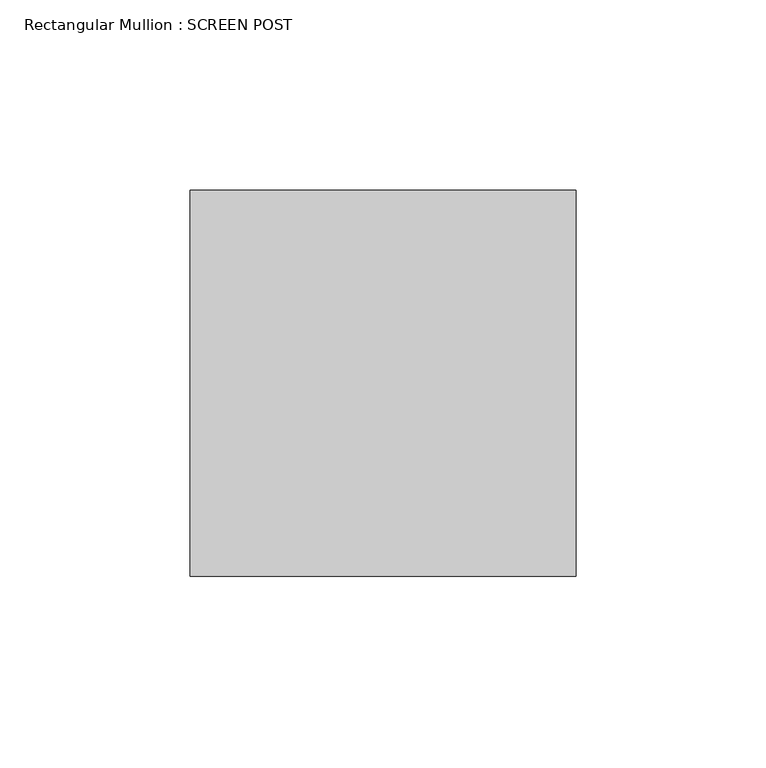
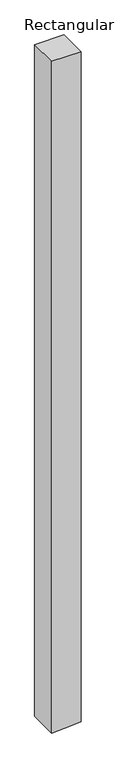
"""IFC4 building model written with IfcOpenShell, lengths in millimetres: member geometry, Rectangular Mullion : SCREEN POST."""

import ifcopenshell
import ifcopenshell.guid

model = None  # the IFC model being written
_history = None  # IfcOwnerHistory: only IFC2X3 demands one
_inside = {}  # id of a spatial element -> (the spatial element, [elements in it])
_under = {}  # id of a project, library or spatial element -> (it, [spatial elements below it])
_declared = {}  # id of a project -> (the project, [libraries it declares])
_typed = {}  # id of a type object -> (the type object, [elements of that type])
_made_of = {}  # id of a material, layer set ... -> (it, [elements and type objects made of it])


def new_model(schema):
    """Start an empty IFC model of exactly this schema.

    Asked for "IFC4X3", IfcOpenShell would pick the latest addendum, in which some entities
    have other attributes; the version numbers below select the first issue.
    IFC2X3 requires an IfcOwnerHistory on every rooted entity: one is made here for all.
    """
    global model, _history
    if schema == "IFC4X3":
        model = ifcopenshell.file(schema_version=(4, 3, 0, 0))
    else:
        model = ifcopenshell.file(schema=schema)
    _inside.clear()
    _under.clear()
    _declared.clear()
    _typed.clear()
    _made_of.clear()
    _history = None
    if model.schema == "IFC2X3":
        org = make("IfcOrganization", Name="unknown")
        user = make(
            "IfcPersonAndOrganization",
            ThePerson=make("IfcPerson", FamilyName="unknown"),
            TheOrganization=org,
        )
        app = make(
            "IfcApplication",
            ApplicationDeveloper=org,
            Version="unknown",
            ApplicationFullName="unknown",
            ApplicationIdentifier="unknown",
        )
        _history = make(
            "IfcOwnerHistory",
            OwningUser=user,
            OwningApplication=app,
            ChangeAction="ADDED",
            CreationDate=0,
        )
    return model


def make(cls, **values):
    """One entity of the class cls with the attributes given. An attribute that is None is left unset."""
    return model.create_entity(
        cls, **{name: value for name, value in values.items() if value is not None}
    )


def rooted(cls, **values):
    """An entity with a GlobalId (a new one), such as an element, a storey or a relation."""
    return make(cls, GlobalId=ifcopenshell.guid.new(), OwnerHistory=_history, **values)


def si_unit(unit_type, name, prefix=None):
    """IfcSIUnit, for example si_unit("LENGTHUNIT", "METRE", prefix="MILLI")."""
    return make("IfcSIUnit", UnitType=unit_type, Prefix=prefix, Name=name)


def assignment(units):
    """IfcUnitAssignment: the units of a project."""
    return None if units is None else make("IfcUnitAssignment", Units=units)


def point(xyz):
    """IfcCartesianPoint."""
    return None if xyz is None else make("IfcCartesianPoint", Coordinates=xyz)


def direction(xyz):
    """IfcDirection."""
    return None if xyz is None else make("IfcDirection", DirectionRatios=xyz)


def frame(location, z_axis=None, x_axis=None):
    """IfcAxis2Placement3D, a coordinate frame: its origin and axes. An axis left out is left unset."""
    return make(
        "IfcAxis2Placement3D",
        Location=point(location),
        Axis=direction(z_axis),
        RefDirection=direction(x_axis),
    )


def origin():
    """The frame at (0, 0, 0) with its axes left unset."""
    return frame((0.0, 0.0, 0.0))


def place(relative_to, where):
    """IfcLocalPlacement: puts the frame where relative to a parent placement (None: the world)."""
    return make(
        "IfcLocalPlacement", PlacementRelTo=relative_to, RelativePlacement=where
    )


def context(
    kind, dimensions, precision=None, world=None, true_north=None, identifier=None
):
    """IfcGeometricRepresentationContext, for example the 3D "Model" context."""
    return make(
        "IfcGeometricRepresentationContext",
        ContextIdentifier=identifier,
        ContextType=kind,
        CoordinateSpaceDimension=dimensions,
        Precision=precision,
        WorldCoordinateSystem=world,
        TrueNorth=true_north,
    )


def project(units=None, contexts=None):
    """IfcProject with its units and contexts."""
    return rooted(
        "IfcProject",
        Name="project",
        RepresentationContexts=contexts,
        UnitsInContext=assignment(units),
    )


def spatial(cls, under=None, at=None, **own):
    """A site, building, storey or space (cls), placed at a placement, below another one or the project."""
    s = rooted(cls, ObjectPlacement=at, **own)
    if under is not None:
        _under.setdefault(under.id(), (under, []))[1].append(s)
    return s


def polyline(points):
    """IfcPolyline through the points."""
    return make("IfcPolyline", Points=[point(p) for p in points])


def outline(outer, holes=None, kind="AREA"):
    """IfcArbitraryClosedProfileDef: a profile drawn as a closed curve; with holes, ...WithVoids."""
    if holes is None:
        return make("IfcArbitraryClosedProfileDef", ProfileType=kind, OuterCurve=outer)
    return make(
        "IfcArbitraryProfileDefWithVoids",
        ProfileType=kind,
        OuterCurve=outer,
        InnerCurves=holes,
    )


def extrude(swept, where, along, depth):
    """IfcExtrudedAreaSolid: the profile swept, set in the frame where, extruded along a direction by depth."""
    return make(
        "IfcExtrudedAreaSolid",
        SweptArea=swept,
        Position=where,
        ExtrudedDirection=direction(along),
        Depth=depth,
    )


def shape(context_of_items, identifier, shape_type, items):
    """IfcShapeRepresentation: the items that make up one representation, for example the "Body"."""
    return make(
        "IfcShapeRepresentation",
        ContextOfItems=context_of_items,
        RepresentationIdentifier=identifier,
        RepresentationType=shape_type,
        Items=items,
    )


def source(mapping_origin, context_of_items, identifier, shape_type, items):
    """IfcRepresentationMap: a shape defined once, which mapped items show again and again."""
    return make(
        "IfcRepresentationMap",
        MappingOrigin=mapping_origin,
        MappedRepresentation=shape(context_of_items, identifier, shape_type, items),
    )


def transform(
    local_origin,
    x_axis=None,
    y_axis=None,
    z_axis=None,
    scale=None,
    scale2=None,
    scale3=None,
    uniform=True,
):
    """IfcCartesianTransformationOperator3D, or its non-uniform kind. x_axis, y_axis, z_axis: its Axis1, 2, 3."""
    if uniform:
        return make(
            "IfcCartesianTransformationOperator3D",
            Axis1=direction(x_axis),
            Axis2=direction(y_axis),
            LocalOrigin=point(local_origin),
            Scale=scale,
            Axis3=direction(z_axis),
        )
    return make(
        "IfcCartesianTransformationOperator3DnonUniform",
        Axis1=direction(x_axis),
        Axis2=direction(y_axis),
        LocalOrigin=point(local_origin),
        Scale=scale,
        Axis3=direction(z_axis),
        Scale2=scale2,
        Scale3=scale3,
    )


def mapped(mapping_source, mapping_target):
    """IfcMappedItem: shows the shape of a source again, moved by a transform."""
    return make(
        "IfcMappedItem", MappingSource=mapping_source, MappingTarget=mapping_target
    )


def made_of(thing, what):
    """Note that an element or type object is made of a material, layer set ...; save() writes the relation."""
    if what is not None:
        _made_of.setdefault(what.id(), (what, []))[1].append(thing)
    return thing


def element(
    cls,
    number,
    at=None,
    inside=None,
    cuts=None,
    type_object=None,
    material=None,
    context=None,
    identifier="Body",
    shape_type=None,
    held_by="IfcProductDefinitionShape",
    body=None,
    shapes=None,
    **own,
):
    """One element of the class cls, such as IfcWall. Its Tag is "e" and its number.

    at: its placement. inside: the storey or other place that contains it. cuts: it is an
    opening in that element (IfcRelVoidsElement). A single representation is given by context,
    identifier, shape_type and body (its items); several are given by shapes. held_by: the class
    of the entity that holds the representations. save() writes the other relations.
    """
    e = rooted(cls, Tag="e%d" % number, ObjectPlacement=at, **own)
    if body is not None:
        shapes = [shape(context, identifier, shape_type, body)]
    if shapes is not None:
        e.Representation = make(held_by, Representations=shapes)
    if inside is not None:
        _inside.setdefault(inside.id(), (inside, []))[1].append(e)
    if cuts is not None:
        rooted(
            "IfcRelVoidsElement", RelatingBuildingElement=cuts, RelatedOpeningElement=e
        )
    if type_object is not None:
        _typed.setdefault(type_object.id(), (type_object, []))[1].append(e)
    return made_of(e, material)


def aggregate(whole, parts):
    """IfcRelAggregates: a whole, such as a stair, and the parts it consists of."""
    return rooted("IfcRelAggregates", RelatingObject=whole, RelatedObjects=parts)


def save(model, path):
    """Write the relations noted so far, then the file.

    IfcRelAggregates (storeys below a building ...), IfcRelContainedInSpatialStructure (elements
    in a storey), IfcRelDefinesByType, IfcRelAssociatesMaterial and IfcRelDeclares: one each for
    every whole, place, type object, material and project.
    """
    for whole, parts in _under.values():
        aggregate(whole, parts)
    for where, things in _inside.values():
        rooted(
            "IfcRelContainedInSpatialStructure",
            RelatedElements=things,
            RelatingStructure=where,
        )
    for kind, things in _typed.values():
        rooted("IfcRelDefinesByType", RelatedObjects=things, RelatingType=kind)
    for what, things in _made_of.values():
        rooted("IfcRelAssociatesMaterial", RelatedObjects=things, RelatingMaterial=what)
    for by, libraries in _declared.values():
        rooted("IfcRelDeclares", RelatingContext=by, RelatedDefinitions=libraries)
    model.write(path)


def rectangular_mullion_screen_post_858415c3(model_context):
    return source(origin(), model_context, "Body", "SweptSolid", [
        extrude(outline(polyline([(0.0, 50.8), (0.0, -50.8), (-2462.5470097, -50.8), (-2459.7638054, -6.3490391), (-2456.1855375, 50.8), (0.0, 50.8)])), frame((0.0, -50.8, 0.0), z_axis=(0.0, 1.0, 0.0), x_axis=(0.0, 0.0, 1.0)), (0.0, 0.0, 1.0), 101.6),
    ])


if __name__ == "__main__":
    model = new_model("IFC4")
    model_context = context("Model", 3, world=origin())
    ifc_project = project(units=[si_unit("LENGTHUNIT", "METRE", prefix="MILLI")], contexts=[model_context])
    site = spatial("IfcSite", under=ifc_project)
    building = spatial("IfcBuilding", under=site)
    placement = place(None, origin())
    rectangular_mullion_screen_post_shape = rectangular_mullion_screen_post_858415c3(model_context)
    element("IfcMember", 1, ObjectType="Rectangular Mullion : SCREEN POST", at=placement, inside=building, context=model_context, shape_type="MappedRepresentation", body=[
        mapped(rectangular_mullion_screen_post_shape, transform((0.0, 0.0, 0.0), x_axis=(1.0, 0.0, 0.0), y_axis=(0.0, 1.0, 0.0), z_axis=(0.0, 0.0, 1.0))),
    ])
    save(model, "model.ifc")

# Revit data of these elements
# Type "Rectangular Mullion : SCREEN POST"
#   built-in parameter 1007304 = 0.333333 (stored number, unit not read)
#   built-in parameter 1007301 = 0.166667 (stored number, unit not read)
#   built-in parameter 1007300 = 0.166667 (stored number, unit not read)
# Element 1 (IfcMember, "Rectangular Mullion : SCREEN POST")
#   Materials on its faces: "SCREEN PORCH FRAMING"
# Materials
#   "SCREEN PORCH FRAMING": class "Wood", colour RGB 164 134 123, transparency 0, Description = "Pinus Echinata", Cost = 0
